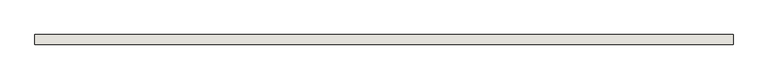
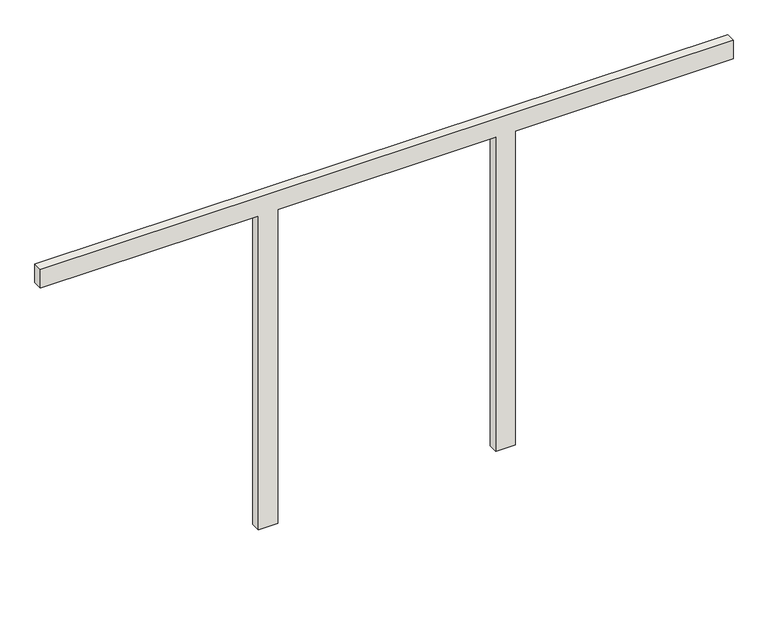
"""IFC4 building model written with IfcOpenShell, lengths in millimetres: wall geometry, 0_3d_modell."""

from ifc_helpers import new_model, si_unit, frame, origin, place, context, project, spatial, polyline, outline, extrude, source, transform, mapped, element, save


def wall_29c5e005(model_context):
    return source(origin(), model_context, "Body", "SweptSolid", [
        extrude(outline(polyline([(2720.0, 0.0), (2720.0, 1783.4), (0.0, 1783.4), (0.0, 1943.4), (2720.0, 1943.4), (2720.0, 3726.7), (0.0, 3726.7), (0.0, 3886.7), (2720.0, 3886.7), (2720.0, 5670.0), (2880.0, 5670.0), (2880.0, 0.0), (2720.0, 0.0)])), frame((0.0, 0.0, 0.0), z_axis=(0.0, 1.0, 0.0), x_axis=(0.0, 0.0, 1.0)), (0.0, 0.0, 1.0), 78.0),
    ])


if __name__ == "__main__":
    model = new_model("IFC4")
    model_context = context("Model", 3, world=origin())
    ifc_project = project(units=[si_unit("LENGTHUNIT", "METRE", prefix="MILLI")], contexts=[model_context])
    site = spatial("IfcSite", under=ifc_project)
    building = spatial("IfcBuilding", under=site)
    placement = place(None, origin())
    wall_shape = wall_29c5e005(model_context)
    element("IfcWall", 1, ObjectType="0_3d_modell", at=placement, inside=building, context=model_context, shape_type="MappedRepresentation", body=[
        mapped(wall_shape, transform((0.0, 0.0, 0.0), x_axis=(1.0, 0.0, 0.0), y_axis=(0.0, 1.0, 0.0), z_axis=(0.0, 0.0, 1.0))),
    ])
    save(model, "model.ifc")

# Revit data of these elements
# Element 1 (IfcWall, "0_3d_modell")
#   Materials on its faces: "glas"
# Materials
#   "glas": class "Unassigned", colour RGB 250 253 254, transparency 0.95
